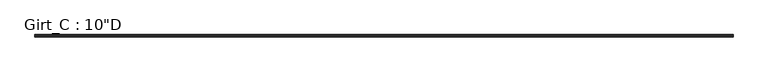
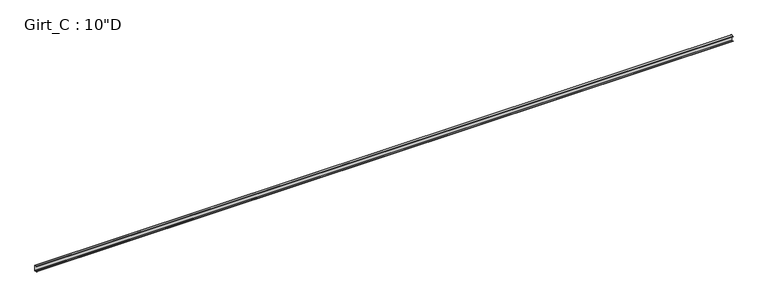
"""IFC4 building model written with IfcOpenShell, lengths in millimetres: beam geometry."""

import ifcopenshell
import ifcopenshell.guid

model = None  # the IFC model being written
_history = None  # IfcOwnerHistory: only IFC2X3 demands one
_inside = {}  # id of a spatial element -> (the spatial element, [elements in it])
_under = {}  # id of a project, library or spatial element -> (it, [spatial elements below it])
_declared = {}  # id of a project -> (the project, [libraries it declares])
_typed = {}  # id of a type object -> (the type object, [elements of that type])
_made_of = {}  # id of a material, layer set ... -> (it, [elements and type objects made of it])


def new_model(schema):
    """Start an empty IFC model of exactly this schema.

    Asked for "IFC4X3", IfcOpenShell would pick the latest addendum, in which some entities
    have other attributes; the version numbers below select the first issue.
    IFC2X3 requires an IfcOwnerHistory on every rooted entity: one is made here for all.
    """
    global model, _history
    if schema == "IFC4X3":
        model = ifcopenshell.file(schema_version=(4, 3, 0, 0))
    else:
        model = ifcopenshell.file(schema=schema)
    _inside.clear()
    _under.clear()
    _declared.clear()
    _typed.clear()
    _made_of.clear()
    _history = None
    if model.schema == "IFC2X3":
        org = make("IfcOrganization", Name="unknown")
        user = make(
            "IfcPersonAndOrganization",
            ThePerson=make("IfcPerson", FamilyName="unknown"),
            TheOrganization=org,
        )
        app = make(
            "IfcApplication",
            ApplicationDeveloper=org,
            Version="unknown",
            ApplicationFullName="unknown",
            ApplicationIdentifier="unknown",
        )
        _history = make(
            "IfcOwnerHistory",
            OwningUser=user,
            OwningApplication=app,
            ChangeAction="ADDED",
            CreationDate=0,
        )
    return model


def make(cls, **values):
    """One entity of the class cls with the attributes given. An attribute that is None is left unset."""
    return model.create_entity(
        cls, **{name: value for name, value in values.items() if value is not None}
    )


def rooted(cls, **values):
    """An entity with a GlobalId (a new one), such as an element, a storey or a relation."""
    return make(cls, GlobalId=ifcopenshell.guid.new(), OwnerHistory=_history, **values)


def si_unit(unit_type, name, prefix=None):
    """IfcSIUnit, for example si_unit("LENGTHUNIT", "METRE", prefix="MILLI")."""
    return make("IfcSIUnit", UnitType=unit_type, Prefix=prefix, Name=name)


def assignment(units):
    """IfcUnitAssignment: the units of a project."""
    return None if units is None else make("IfcUnitAssignment", Units=units)


def point(xyz):
    """IfcCartesianPoint."""
    return None if xyz is None else make("IfcCartesianPoint", Coordinates=xyz)


def direction(xyz):
    """IfcDirection."""
    return None if xyz is None else make("IfcDirection", DirectionRatios=xyz)


def frame(location, z_axis=None, x_axis=None):
    """IfcAxis2Placement3D, a coordinate frame: its origin and axes. An axis left out is left unset."""
    return make(
        "IfcAxis2Placement3D",
        Location=point(location),
        Axis=direction(z_axis),
        RefDirection=direction(x_axis),
    )


def frame_2d(location, x_axis=None):
    """IfcAxis2Placement2D, a coordinate frame in the plane: its origin and x axis."""
    return make(
        "IfcAxis2Placement2D", Location=point(location), RefDirection=direction(x_axis)
    )


def origin():
    """The frame at (0, 0, 0) with its axes left unset."""
    return frame((0.0, 0.0, 0.0))


def place(relative_to, where):
    """IfcLocalPlacement: puts the frame where relative to a parent placement (None: the world)."""
    return make(
        "IfcLocalPlacement", PlacementRelTo=relative_to, RelativePlacement=where
    )


def context(
    kind, dimensions, precision=None, world=None, true_north=None, identifier=None
):
    """IfcGeometricRepresentationContext, for example the 3D "Model" context."""
    return make(
        "IfcGeometricRepresentationContext",
        ContextIdentifier=identifier,
        ContextType=kind,
        CoordinateSpaceDimension=dimensions,
        Precision=precision,
        WorldCoordinateSystem=world,
        TrueNorth=true_north,
    )


def project(units=None, contexts=None):
    """IfcProject with its units and contexts."""
    return rooted(
        "IfcProject",
        Name="project",
        RepresentationContexts=contexts,
        UnitsInContext=assignment(units),
    )


def spatial(cls, under=None, at=None, **own):
    """A site, building, storey or space (cls), placed at a placement, below another one or the project."""
    s = rooted(cls, ObjectPlacement=at, **own)
    if under is not None:
        _under.setdefault(under.id(), (under, []))[1].append(s)
    return s


def polyline(points):
    """IfcPolyline through the points."""
    return make("IfcPolyline", Points=[point(p) for p in points])


def circle_curve(where, radius):
    """IfcCircle in the frame where."""
    return make("IfcCircle", Position=where, Radius=radius)


def trimmed(basis, trim1, trim2, sense, master):
    """IfcTrimmedCurve: the piece of a basis curve between two trims."""
    return make(
        "IfcTrimmedCurve",
        BasisCurve=basis,
        Trim1=trim1,
        Trim2=trim2,
        SenseAgreement=sense,
        MasterRepresentation=master,
    )


def segment(curve, same_sense, transition):
    """IfcCompositeCurveSegment."""
    return make(
        "IfcCompositeCurveSegment",
        Transition=transition,
        SameSense=same_sense,
        ParentCurve=curve,
    )


def composite_curve(segments, self_intersect=None):
    """IfcCompositeCurve: segments joined end to end."""
    return make("IfcCompositeCurve", Segments=segments, SelfIntersect=self_intersect)


def outline(outer, holes=None, kind="AREA"):
    """IfcArbitraryClosedProfileDef: a profile drawn as a closed curve; with holes, ...WithVoids."""
    if holes is None:
        return make("IfcArbitraryClosedProfileDef", ProfileType=kind, OuterCurve=outer)
    return make(
        "IfcArbitraryProfileDefWithVoids",
        ProfileType=kind,
        OuterCurve=outer,
        InnerCurves=holes,
    )


def extrude(swept, where, along, depth):
    """IfcExtrudedAreaSolid: the profile swept, set in the frame where, extruded along a direction by depth."""
    return make(
        "IfcExtrudedAreaSolid",
        SweptArea=swept,
        Position=where,
        ExtrudedDirection=direction(along),
        Depth=depth,
    )


def shape(context_of_items, identifier, shape_type, items):
    """IfcShapeRepresentation: the items that make up one representation, for example the "Body"."""
    return make(
        "IfcShapeRepresentation",
        ContextOfItems=context_of_items,
        RepresentationIdentifier=identifier,
        RepresentationType=shape_type,
        Items=items,
    )


def source(mapping_origin, context_of_items, identifier, shape_type, items):
    """IfcRepresentationMap: a shape defined once, which mapped items show again and again."""
    return make(
        "IfcRepresentationMap",
        MappingOrigin=mapping_origin,
        MappedRepresentation=shape(context_of_items, identifier, shape_type, items),
    )


def transform(
    local_origin,
    x_axis=None,
    y_axis=None,
    z_axis=None,
    scale=None,
    scale2=None,
    scale3=None,
    uniform=True,
):
    """IfcCartesianTransformationOperator3D, or its non-uniform kind. x_axis, y_axis, z_axis: its Axis1, 2, 3."""
    if uniform:
        return make(
            "IfcCartesianTransformationOperator3D",
            Axis1=direction(x_axis),
            Axis2=direction(y_axis),
            LocalOrigin=point(local_origin),
            Scale=scale,
            Axis3=direction(z_axis),
        )
    return make(
        "IfcCartesianTransformationOperator3DnonUniform",
        Axis1=direction(x_axis),
        Axis2=direction(y_axis),
        LocalOrigin=point(local_origin),
        Scale=scale,
        Axis3=direction(z_axis),
        Scale2=scale2,
        Scale3=scale3,
    )


def mapped(mapping_source, mapping_target):
    """IfcMappedItem: shows the shape of a source again, moved by a transform."""
    return make(
        "IfcMappedItem", MappingSource=mapping_source, MappingTarget=mapping_target
    )


def made_of(thing, what):
    """Note that an element or type object is made of a material, layer set ...; save() writes the relation."""
    if what is not None:
        _made_of.setdefault(what.id(), (what, []))[1].append(thing)
    return thing


def element(
    cls,
    number,
    at=None,
    inside=None,
    cuts=None,
    type_object=None,
    material=None,
    context=None,
    identifier="Body",
    shape_type=None,
    held_by="IfcProductDefinitionShape",
    body=None,
    shapes=None,
    **own,
):
    """One element of the class cls, such as IfcWall. Its Tag is "e" and its number.

    at: its placement. inside: the storey or other place that contains it. cuts: it is an
    opening in that element (IfcRelVoidsElement). A single representation is given by context,
    identifier, shape_type and body (its items); several are given by shapes. held_by: the class
    of the entity that holds the representations. save() writes the other relations.
    """
    e = rooted(cls, Tag="e%d" % number, ObjectPlacement=at, **own)
    if body is not None:
        shapes = [shape(context, identifier, shape_type, body)]
    if shapes is not None:
        e.Representation = make(held_by, Representations=shapes)
    if inside is not None:
        _inside.setdefault(inside.id(), (inside, []))[1].append(e)
    if cuts is not None:
        rooted(
            "IfcRelVoidsElement", RelatingBuildingElement=cuts, RelatedOpeningElement=e
        )
    if type_object is not None:
        _typed.setdefault(type_object.id(), (type_object, []))[1].append(e)
    return made_of(e, material)


def aggregate(whole, parts):
    """IfcRelAggregates: a whole, such as a stair, and the parts it consists of."""
    return rooted("IfcRelAggregates", RelatingObject=whole, RelatedObjects=parts)


def save(model, path):
    """Write the relations noted so far, then the file.

    IfcRelAggregates (storeys below a building ...), IfcRelContainedInSpatialStructure (elements
    in a storey), IfcRelDefinesByType, IfcRelAssociatesMaterial and IfcRelDeclares: one each for
    every whole, place, type object, material and project.
    """
    for whole, parts in _under.values():
        aggregate(whole, parts)
    for where, things in _inside.values():
        rooted(
            "IfcRelContainedInSpatialStructure",
            RelatedElements=things,
            RelatingStructure=where,
        )
    for kind, things in _typed.values():
        rooted("IfcRelDefinesByType", RelatedObjects=things, RelatingType=kind)
    for what, things in _made_of.values():
        rooted("IfcRelAssociatesMaterial", RelatedObjects=things, RelatingMaterial=what)
    for by, libraries in _declared.values():
        rooted("IfcRelDeclares", RelatingContext=by, RelatedDefinitions=libraries)
    model.write(path)


def beam_8a3f25ab(model_context):
    return source(origin(), model_context, "Body", "SweptSolid", [
        extrude(outline(composite_curve([segment(polyline([(-87.5109375, 127.0), (-3.3734375, 127.0)]), True, "CONTINUOUS"), segment(trimmed(circle_curve(frame_2d((-3.3734375, 122.2375)), 4.7625), [point((-3.3734375, 127.0))], [point((1.3890625, 122.2375))], False, "CARTESIAN"), True, "CONTINUOUS"), segment(polyline([(1.3890625, 122.2375), (1.3890625, -122.2375)]), True, "CONTINUOUS"), segment(trimmed(circle_curve(frame_2d((-3.3734375, -122.2375)), 4.7625), [point((1.3890625, -122.2375))], [point((-3.3734375, -127.0))], False, "CARTESIAN"), True, "CONTINUOUS"), segment(polyline([(-3.3734375, -127.0), (-87.5109375, -127.0), (-99.7792647, -112.379177), (-97.6510975, -110.5934327), (-86.2154765, -124.221875), (-3.2694106, -124.221875)]), True, "CONTINUOUS"), segment(trimmed(circle_curve(frame_2d((-3.3748024, -122.2389339)), 1.9857399), [point((-3.2694106, -124.221875))], [point((-1.3890625, -122.2389339))], True, "CARTESIAN"), True, "CONTINUOUS"), segment(polyline([(-1.3890625, -122.2389339), (-1.3890625, 122.2381931)]), True, "CONTINUOUS"), segment(trimmed(circle_curve(frame_2d((-3.3741066, 122.2381931)), 1.9850441), [point((-1.3890625, 122.2381931))], [point((-3.3005807, 124.221875))], True, "CARTESIAN"), True, "CONTINUOUS"), segment(polyline([(-3.3005807, 124.221875), (-86.2154765, 124.221875), (-97.6278742, 110.621109), (-99.7560415, 112.4068534), (-87.5109375, 127.0)]), True, "CONTINUOUS")], self_intersect=False)), frame((-15567.025, 0.0, 0.0), z_axis=(1.0, 0.0, 0.0), x_axis=(0.0, 1.0, 0.0)), (0.0, 0.0, 1.0), 31127.7),
    ])


if __name__ == "__main__":
    model = new_model("IFC4")
    model_context = context("Model", 3, world=origin())
    ifc_project = project(units=[si_unit("LENGTHUNIT", "METRE", prefix="MILLI")], contexts=[model_context])
    site = spatial("IfcSite", under=ifc_project)
    building = spatial("IfcBuilding", under=site)
    placement = place(None, origin())
    beam_shape = beam_8a3f25ab(model_context)
    element("IfcBeam", 1, ObjectType="Girt_C : 10\"D", at=placement, inside=building, context=model_context, shape_type="MappedRepresentation", body=[
        mapped(beam_shape, transform((0.0, 0.0, 0.0), x_axis=(1.0, 0.0, 0.0), y_axis=(0.0, 1.0, 0.0), z_axis=(0.0, 0.0, 1.0))),
    ])
    save(model, "model.ifc")

# Revit data of these elements
# Type "Girt_C : 10\"D"
#   half leg = 0' - 1 3/4"
#   Web_Thickness = 0' - 0 7/64"
#   Length [instance default] = 10' - 0"
#   Leg_1 = 0' - 3 1/2"
#   Height = 0' - 10"
#   Structural Material [instance default] = none
# Element 1 (IfcBeam, "Girt_C : 10\"D")
#   Structural Material = STRUCTURAL STEEL - SEE STRUCT. DWGS
#   Materials on its faces: "STRUCTURAL STEEL - SEE STRUCT. DWGS"
# Materials
#   "STRUCTURAL STEEL - SEE STRUCT. DWGS": class "Metal", colour RGB 137 146 153, transparency 0, Description = "Steel, mill finish", Cost = 0
